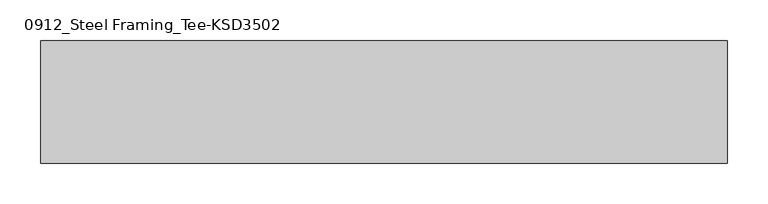
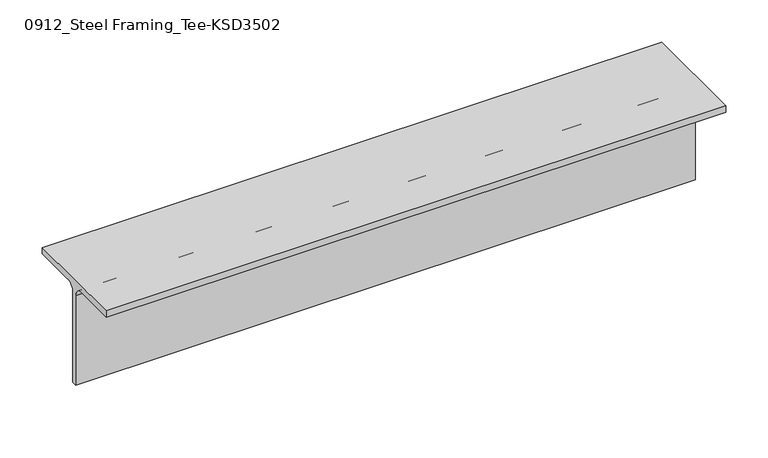
"""IFC4 building model written with IfcOpenShell, lengths in millimetres: member geometry, 0912_Steel Framing_Tee-KSD3502 : H_SB_ASB_CT-150x150x6.5x9."""

from ifc_helpers import new_model, si_unit, point, frame, frame_2d, origin, place, context, project, spatial, polyline, circle_curve, trimmed, segment, composite_curve, outline, extrude, source, transform, mapped, element, save


def member_0912_steel_framing_tee_ksd3502_6e3fb3f0(model_context):
    return source(origin(), model_context, "Body", "SweptSolid", [
        extrude(outline(composite_curve([segment(polyline([(75.0, 75.0), (75.0, 66.0), (16.25, 66.0)]), True, "CONTINUOUS"), segment(trimmed(circle_curve(frame_2d((16.25, 53.0)), 13.0), [point((16.25, 66.0))], [point((3.25, 53.0))], True, "CARTESIAN"), True, "CONTINUOUS"), segment(polyline([(3.25, 53.0), (3.25, -75.0), (-3.25, -75.0), (-3.25, 53.0)]), True, "CONTINUOUS"), segment(trimmed(circle_curve(frame_2d((-16.25, 53.0)), 13.0), [point((-3.25, 53.0))], [point((-16.25, 66.0))], True, "CARTESIAN"), True, "CONTINUOUS"), segment(polyline([(-16.25, 66.0), (-75.0, 66.0), (-75.0, 75.0), (75.0, 75.0)]), True, "CONTINUOUS")], self_intersect=False)), frame((-341.5, 0.0, 0.0), z_axis=(1.0, 0.0, 0.0), x_axis=(0.0, 1.0, 0.0)), (0.0, 0.0, 1.0), 841.5),
    ])


if __name__ == "__main__":
    model = new_model("IFC4")
    model_context = context("Model", 3, world=origin())
    ifc_project = project(units=[si_unit("LENGTHUNIT", "METRE", prefix="MILLI")], contexts=[model_context])
    site = spatial("IfcSite", under=ifc_project)
    building = spatial("IfcBuilding", under=site)
    placement = place(None, origin())
    member_0912_steel_framing_tee_ksd3502_shape = member_0912_steel_framing_tee_ksd3502_6e3fb3f0(model_context)
    element("IfcMember", 1, ObjectType="0912_Steel Framing_Tee-KSD3502 : H_SB_ASB_CT-150x150x6.5x9", at=placement, inside=building, context=model_context, shape_type="MappedRepresentation", body=[
        mapped(member_0912_steel_framing_tee_ksd3502_shape, transform((0.0, 0.0, 0.0), x_axis=(1.0, 0.0, 0.0), y_axis=(0.0, 1.0, 0.0), z_axis=(0.0, 0.0, 1.0))),
    ])
    save(model, "model.ifc")

# Revit data of these elements
# Type "0912_Steel Framing_Tee-KSD3502 : H_SB_ASB_CT-150x150x6.5x9"
#   H_WM Code_1 = "S01AA003-00001 | Main Steel Structure Fabrication Work | Shelter/Building | Light Steel - Standard (30KG/M>Weight) | Material: (   )"
#   H_WM Code_2 = "S03AA029-00001 | Main Steel Structure Erection Work | Shelter/Building | Light Steel (30KG/M>Weight) | Material: (   )"
#   H_WM Code_3 = "S01AA010-00001 | Main Steel Structure Fabrication Work | Shelter/Building | Steel Painting/Coating | for Non-Fireproofed Steel Surface, Surface Preparation, Primer, Second & Final Coat | Material: (   )"
#   H_Q'ty Cal Type Tag = "SB-Q2"
#   Width = 15.0 cm
#   Web Thickness = 0.65 cm
#   Web Fillet = 1.3 cm
#   Section Area = 23.39 cm²
#   Perimeter = 0.60 m²/m
#   Nominal Weight = 18.40 kgf/m
#   Height = 15.0 cm
#   Flange Thickness = 0.9 cm
#   Centroid Vertical = 7.5 cm
#   Centroid Horizontal = 7.5 cm
#   Length [instance default] = 1.5000 m
#   Structural Material [instance default] = Steel, 45-345
#   Warping Constant = (empty or 0)
#   Torsional Moment of Inertia = 0
#   Section Name Key = ""
#   Plastic Modulus weak axis = 0
#   Plastic Modulus strong axis = 0
#   Moment of Inertia weak axis = 0
#   Moment of Inertia strong axis = 0
#   Elastic Modulus weak axis = 0
#   Elastic Modulus strong axis = 0
#   Bolt Spacing = 0
#   Assembly Code = ""
# Element 1 (IfcMember, "0912_Steel Framing_Tee-KSD3502 : H_SB_ASB_CT-150x150x6.5x9")
#   Structural Material = none
# Materials
#   "Steel, 45-345": class "Metal", colour RGB 189 187 185, transparency 0, Description = "Steel 345 MPa", Cost = 0
